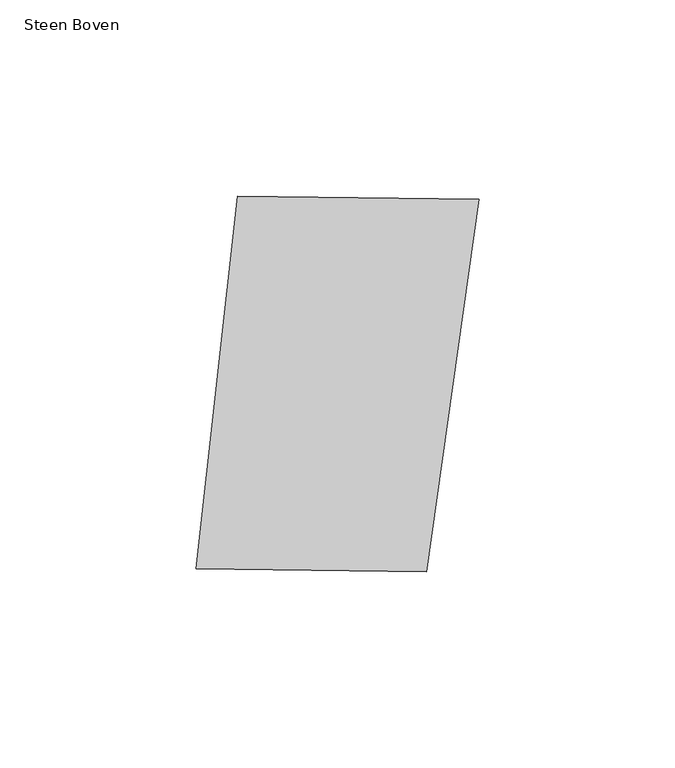
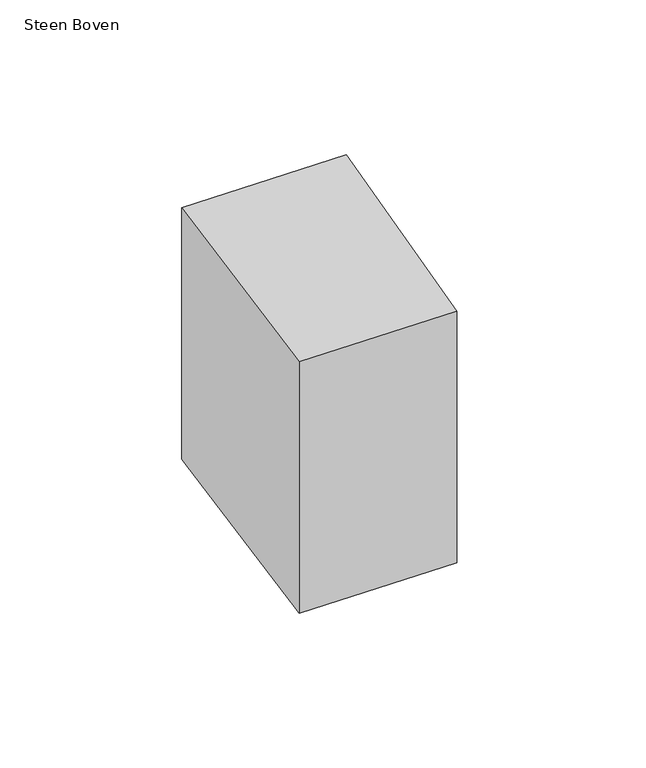
"""IFC4 building model written with IfcOpenShell, lengths in millimetres: proxy geometry, 00_GMA_steen_versie_4 : Steen Boven."""

from ifc_helpers import new_model, si_unit, origin, origin_with_axes, place, context, project, spatial, polyline, outline, extrude, source, transform, mapped, element, save


def steen_boven_33a2fb8a(model_context):
    return source(origin(), model_context, "Body", "SweptSolid", [
        extrude(outline(polyline([(107.5673675, 118.576131), (94.2352564, 23.6861521), (35.5279268, 24.3876501), (46.1430117, 119.2957835), (107.5673675, 118.576131)])), origin_with_axes(), (0.0, 0.0, 1.0), 100.0),
    ])


if __name__ == "__main__":
    model = new_model("IFC4")
    model_context = context("Model", 3, world=origin())
    ifc_project = project(units=[si_unit("LENGTHUNIT", "METRE", prefix="MILLI")], contexts=[model_context])
    site = spatial("IfcSite", under=ifc_project)
    building = spatial("IfcBuilding", under=site)
    placement = place(None, origin())
    steen_boven_shape = steen_boven_33a2fb8a(model_context)
    element("IfcBuildingElementProxy", 1, Name="00_GMA_steen_versie_4 : Steen Boven", ObjectType="00_GMA_steen_versie_4 : Steen Boven", at=placement, inside=building, context=model_context, shape_type="MappedRepresentation", body=[
        mapped(steen_boven_shape, transform((0.0, 0.0, 0.0), x_axis=(1.0, 0.0, 0.0), y_axis=(0.0, 1.0, 0.0), z_axis=(0.0, 0.0, 1.0))),
    ])
    save(model, "model.ifc")

# Revit data of these elements
# Type "00_GMA_steen_versie_4 : Steen Boven"
#   StootVoegHalfBoven [instance default] = 5 mm
#   StootVoegHalf [instance default] = 5 mm
#   StootVoegBreedteOnder = 10 mm
#   StootVoegBreedteBoven = 10 mm
#   Steendikte = 100 mm
#   LintVoegOnderHalf = 5 mm
#   LintVoegOnder = 10 mm
#   LintVoegBovenHalf = 0 mm
#   LintVoegBoven = 0 mm
#   materiaal = none
#   MateriaalVoeg = none
#   Default Elevation = 0
